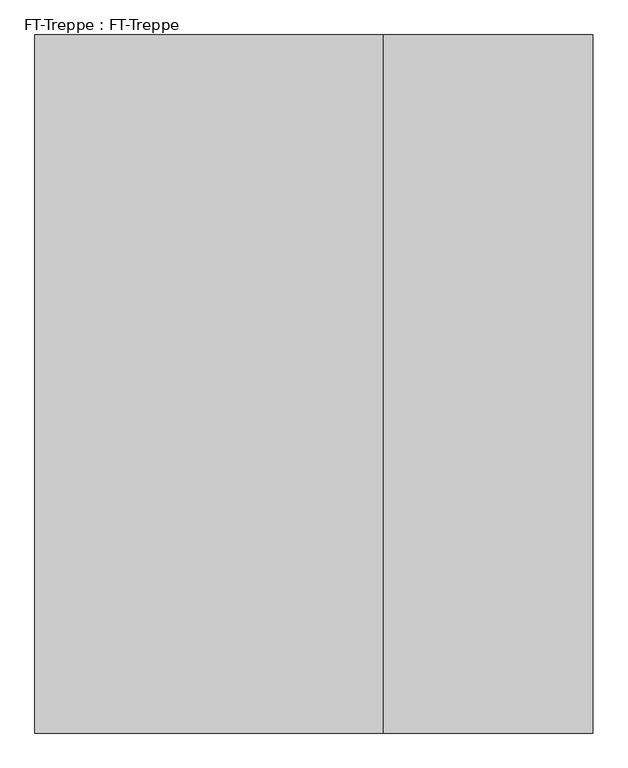
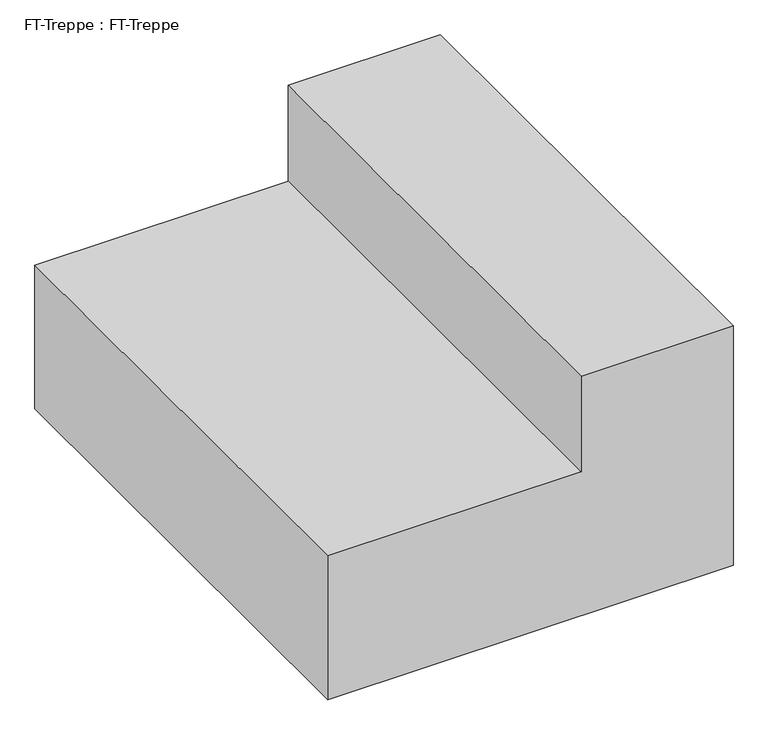
"""IFC4 building model written with IfcOpenShell, lengths in millimetres: stair geometry, FT-Treppe : FT-Treppe."""

from ifc_helpers import new_model, si_unit, frame, origin, place, context, project, spatial, polyline, outline, extrude, source, transform, mapped, element, save


def ft_treppe_ft_treppe_1f8feaef(model_context):
    return source(origin(), model_context, "Body", "SweptSolid", [
        extrude(outline(polyline([(-860.9044, 5581.873984), (-360.9044, 5581.873984), (-360.9044, 5281.873984), (-560.9044, 5281.873984), (-560.9044, 4781.873984), (-860.9044, 4781.873984), (-860.9044, 5581.873984)])), frame((0.0, 8969.5273241, 0.0), z_axis=(0.0, 1.0, 0.0), x_axis=(0.0, 0.0, 1.0)), (0.0, 0.0, 1.0), 999.9999955),
    ])


if __name__ == "__main__":
    model = new_model("IFC4")
    model_context = context("Model", 3, world=origin())
    ifc_project = project(units=[si_unit("LENGTHUNIT", "METRE", prefix="MILLI")], contexts=[model_context])
    site = spatial("IfcSite", under=ifc_project)
    building = spatial("IfcBuilding", under=site)
    placement = place(None, origin())
    ft_treppe_ft_treppe_shape = ft_treppe_ft_treppe_1f8feaef(model_context)
    element("IfcStair", 1, ObjectType="FT-Treppe : FT-Treppe", at=placement, inside=building, context=model_context, shape_type="MappedRepresentation", body=[
        mapped(ft_treppe_ft_treppe_shape, transform((0.0, 0.0, 0.0), x_axis=(1.0, 0.0, 0.0), y_axis=(0.0, 1.0, 0.0), z_axis=(0.0, 0.0, 1.0))),
    ])
    save(model, "model.ifc")

# Revit data of these elements
# Element 1 (IfcStair, "FT-Treppe : FT-Treppe")
#   Materials on its faces: "Ortbeton - bewehrt"
# Materials
#   "Ortbeton - bewehrt": class "Beton", colour RGB 247 247 247, transparency 0, Description = "Ortbeton - bewehrt", Cost = 0
